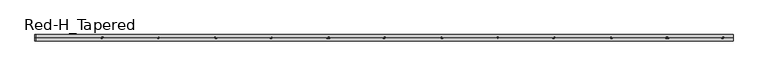
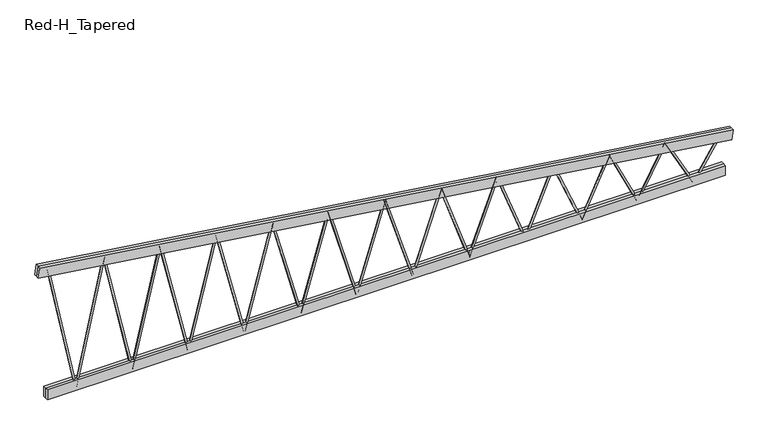
"""IFC4 building model written with IfcOpenShell, lengths in millimetres: beam geometry, Construction_Frames_RedBuilt_Openweb_Red-H_Tapered : Red-H_Tapered."""

from ifc_helpers import new_model, si_unit, point, frame, origin, origin_2d, place, context, project, spatial, polyline, circle_curve, trimmed, segment, composite_curve, outline, extrude, source, transform, mapped, element, save


def red_h_tapered_d8ccadf6(model_context):
    return source(origin(), model_context, "Body", "SweptSolid", [
        extrude(outline(composite_curve([segment(trimmed(circle_curve(origin_2d(), 12.7), [point((0.0, -12.7000001))], [point((0.0, 12.7))], False, "CARTESIAN"), True, "CONTINUOUS"), segment(trimmed(circle_curve(origin_2d(), 12.7), [point((0.0, 12.7))], [point((0.0, -12.7000001))], False, "CARTESIAN"), True, "CONTINUOUS")], self_intersect=False)), frame((-373.9223958, 0.0, -367.0101562), z_axis=(-0.2781430726229013, 0.0, 0.9605396562099305), x_axis=(0.0, -1.0, 0.0)), (0.0, 0.0, 1.0), 1344.3527186),
        extrude(outline(composite_curve([segment(trimmed(circle_curve(origin_2d(), 12.7), [point((0.0, 12.7))], [point((0.0, -12.7))], False, "CARTESIAN"), True, "CONTINUOUS"), segment(trimmed(circle_curve(origin_2d(), 12.7), [point((0.0, -12.7))], [point((0.0, 12.7))], False, "CARTESIAN"), True, "CONTINUOUS")], self_intersect=False)), frame((-1121.7671875, 0.0, -367.0101562), z_axis=(0.27814307262290183, 0.0, 0.9605396562099304), x_axis=(0.0, -1.0, 0.0)), (0.0, 0.0, 1.0), 1344.3527186),
        extrude(outline(composite_curve([segment(trimmed(circle_curve(origin_2d(), 12.7), [point((0.0, -12.7))], [point((0.0, 12.7))], False, "CARTESIAN"), True, "CONTINUOUS"), segment(trimmed(circle_curve(origin_2d(), 12.7), [point((0.0, 12.7))], [point((0.0, -12.7))], False, "CARTESIAN"), True, "CONTINUOUS")], self_intersect=False)), frame((-1121.7671875, 0.0, -367.0101562), z_axis=(-0.259370176676437, 0.0, 0.9657779824839837), x_axis=(0.0, -1.0, 0.0)), (0.0, 0.0, 1.0), 1441.655323),
        extrude(outline(composite_curve([segment(trimmed(circle_curve(origin_2d(), 12.7), [point((0.0, -12.6999999))], [point((0.0, 12.7))], False, "CARTESIAN"), True, "CONTINUOUS"), segment(trimmed(circle_curve(origin_2d(), 12.7), [point((0.0, 12.7))], [point((0.0, -12.6999999))], False, "CARTESIAN"), True, "CONTINUOUS")], self_intersect=False)), frame((-1869.6119792, 0.0, -367.0101562), z_axis=(0.2593701766764403, 0.0, 0.9657779824839828), x_axis=(0.0, -1.0, 0.0)), (0.0, 0.0, 1.0), 1441.655323),
        extrude(outline(composite_curve([segment(trimmed(circle_curve(origin_2d(), 12.7), [point((0.0, 12.7))], [point((0.0, -12.7))], False, "CARTESIAN"), True, "CONTINUOUS"), segment(trimmed(circle_curve(origin_2d(), 12.7), [point((0.0, -12.7))], [point((0.0, 12.7))], False, "CARTESIAN"), True, "CONTINUOUS")], self_intersect=False)), frame((-1869.6119792, 0.0, -367.0101562), z_axis=(-0.24289567030274667, 0.0, 0.970052417835335), x_axis=(0.0, -1.0, 0.0)), (0.0, 0.0, 1.0), 1539.4362335),
        extrude(outline(composite_curve([segment(trimmed(circle_curve(origin_2d(), 12.7), [point((0.0, -12.7))], [point((0.0, 12.7))], False, "CARTESIAN"), True, "CONTINUOUS"), segment(trimmed(circle_curve(origin_2d(), 12.7), [point((0.0, 12.7))], [point((0.0, -12.7))], False, "CARTESIAN"), True, "CONTINUOUS")], self_intersect=False)), frame((-2617.4567708, 0.0, -367.0101562), z_axis=(0.24289567030274511, 0.0, 0.9700524178353355), x_axis=(0.0, -1.0, 0.0)), (0.0, 0.0, 1.0), 1539.4362335),
        extrude(outline(composite_curve([segment(trimmed(circle_curve(origin_2d(), 12.7), [point((0.0, 12.6999999))], [point((0.0, -12.7))], False, "CARTESIAN"), True, "CONTINUOUS"), segment(trimmed(circle_curve(origin_2d(), 12.7), [point((0.0, -12.7))], [point((0.0, 12.6999999))], False, "CARTESIAN"), True, "CONTINUOUS")], self_intersect=False)), frame((-2617.4567708, 0.0, -367.0101562), z_axis=(-0.2283342477198344, 0.0, 0.9735828014700225), x_axis=(0.0, -1.0, 0.0)), (0.0, 0.0, 1.0), 1637.6097741),
        extrude(outline(composite_curve([segment(trimmed(circle_curve(origin_2d(), 12.7), [point((0.0, -12.7))], [point((0.0, 12.7))], False, "CARTESIAN"), True, "CONTINUOUS"), segment(trimmed(circle_curve(origin_2d(), 12.7), [point((0.0, 12.7))], [point((0.0, -12.7))], False, "CARTESIAN"), True, "CONTINUOUS")], self_intersect=False)), frame((-3365.3015625, 0.0, -367.0101562), z_axis=(0.22833424771983904, 0.0, 0.9735828014700214), x_axis=(0.0, -1.0, 0.0)), (0.0, 0.0, 1.0), 1637.6097741),
        extrude(outline(composite_curve([segment(trimmed(circle_curve(origin_2d(), 12.7), [point((0.0, 12.7))], [point((0.0, -12.7))], False, "CARTESIAN"), True, "CONTINUOUS"), segment(trimmed(circle_curve(origin_2d(), 12.7), [point((0.0, -12.7))], [point((0.0, 12.7))], False, "CARTESIAN"), True, "CONTINUOUS")], self_intersect=False)), frame((-3365.3015625, 0.0, -367.0101562), z_axis=(-0.215379519884342, 0.0, 0.9765304206292759), x_axis=(0.0, -1.0, 0.0)), (0.0, 0.0, 1.0), 1736.1093387),
        extrude(outline(composite_curve([segment(trimmed(circle_curve(origin_2d(), 12.7), [point((0.0, -12.7))], [point((0.0, 12.7000001))], False, "CARTESIAN"), True, "CONTINUOUS"), segment(trimmed(circle_curve(origin_2d(), 12.7), [point((0.0, 12.7000001))], [point((0.0, -12.7))], False, "CARTESIAN"), True, "CONTINUOUS")], self_intersect=False)), frame((-4113.1463542, 0.0, -367.0101562), z_axis=(0.21537951988434104, 0.0, 0.9765304206292761), x_axis=(0.0, -1.0, 0.0)), (0.0, 0.0, 1.0), 1736.1093387),
        extrude(outline(composite_curve([segment(trimmed(circle_curve(origin_2d(), 12.7), [point((0.0, 12.7))], [point((0.0, -12.7))], False, "CARTESIAN"), True, "CONTINUOUS"), segment(trimmed(circle_curve(origin_2d(), 12.7), [point((0.0, -12.7))], [point((0.0, 12.7))], False, "CARTESIAN"), True, "CONTINUOUS")], self_intersect=False)), frame((-4113.1463542, 0.0, -367.0101562), z_axis=(-0.20378548023403467, 0.0, 0.9790155657831922), x_axis=(0.0, -1.0, 0.0)), (0.0, 0.0, 1.0), 1834.8824234),
        extrude(outline(composite_curve([segment(trimmed(circle_curve(origin_2d(), 12.7), [point((0.0, 12.7))], [point((0.0, -12.7))], False, "CARTESIAN"), True, "CONTINUOUS"), segment(trimmed(circle_curve(origin_2d(), 12.7), [point((0.0, -12.7))], [point((0.0, 12.7))], False, "CARTESIAN"), True, "CONTINUOUS")], self_intersect=False)), frame((4113.1463542, 0.0, -367.0101562), z_axis=(0.5390888753862533, 0.0, 0.8422488850896657), x_axis=(0.0, -1.0, 0.0)), (0.0, 0.0, 1.0), 693.6192025),
        extrude(outline(composite_curve([segment(trimmed(circle_curve(origin_2d(), 12.7), [point((0.0, -12.7))], [point((0.0, 12.6999999))], False, "CARTESIAN"), True, "CONTINUOUS"), segment(trimmed(circle_curve(origin_2d(), 12.7), [point((0.0, 12.6999999))], [point((0.0, -12.7))], False, "CARTESIAN"), True, "CONTINUOUS")], self_intersect=False)), frame((4113.1463542, 0.0, -367.0101562), z_axis=(-0.47901881060106194, 0.0, 0.8778046360610908), x_axis=(0.0, -1.0, 0.0)), (0.0, 0.0, 1.0), 780.6006519),
        extrude(outline(composite_curve([segment(trimmed(circle_curve(origin_2d(), 12.7), [point((0.0, 12.7))], [point((0.0, -12.7))], False, "CARTESIAN"), True, "CONTINUOUS"), segment(trimmed(circle_curve(origin_2d(), 12.7), [point((0.0, -12.7))], [point((0.0, 12.7))], False, "CARTESIAN"), True, "CONTINUOUS")], self_intersect=False)), frame((3365.3015625, 0.0, -367.0101562), z_axis=(0.4790188106010647, 0.0, 0.8778046360610893), x_axis=(0.0, -1.0, 0.0)), (0.0, 0.0, 1.0), 780.6006519),
        extrude(outline(composite_curve([segment(trimmed(circle_curve(origin_2d(), 12.7), [point((0.0, -12.7))], [point((0.0, 12.7))], False, "CARTESIAN"), True, "CONTINUOUS"), segment(trimmed(circle_curve(origin_2d(), 12.7), [point((0.0, 12.7))], [point((0.0, -12.7))], False, "CARTESIAN"), True, "CONTINUOUS")], self_intersect=False)), frame((3365.3015625, 0.0, -367.0101562), z_axis=(-0.4294909226192341, 0.0, 0.9030711751504856), x_axis=(0.0, -1.0, 0.0)), (0.0, 0.0, 1.0), 870.6176921),
        extrude(outline(composite_curve([segment(trimmed(circle_curve(origin_2d(), 12.7), [point((0.0, 12.7000001))], [point((0.0, -12.7))], False, "CARTESIAN"), True, "CONTINUOUS"), segment(trimmed(circle_curve(origin_2d(), 12.7), [point((0.0, -12.7))], [point((0.0, 12.7000001))], False, "CARTESIAN"), True, "CONTINUOUS")], self_intersect=False)), frame((2617.4567708, 0.0, -367.0101562), z_axis=(0.42949092261923544, 0.0, 0.903071175150485), x_axis=(0.0, -1.0, 0.0)), (0.0, 0.0, 1.0), 870.6176921),
        extrude(outline(composite_curve([segment(trimmed(circle_curve(origin_2d(), 12.7), [point((0.0, -12.7))], [point((0.0, 12.7))], False, "CARTESIAN"), True, "CONTINUOUS"), segment(trimmed(circle_curve(origin_2d(), 12.7), [point((0.0, 12.7))], [point((0.0, -12.7))], False, "CARTESIAN"), True, "CONTINUOUS")], self_intersect=False)), frame((2617.4567708, 0.0, -367.0101562), z_axis=(-0.3883619744047195, 0.0, 0.9215069054741087), x_axis=(0.0, -1.0, 0.0)), (0.0, 0.0, 1.0), 962.8192781),
        extrude(outline(composite_curve([segment(trimmed(circle_curve(origin_2d(), 12.7), [point((0.0, 12.7))], [point((0.0, -12.7))], False, "CARTESIAN"), True, "CONTINUOUS"), segment(trimmed(circle_curve(origin_2d(), 12.7), [point((0.0, -12.7))], [point((0.0, 12.7))], False, "CARTESIAN"), True, "CONTINUOUS")], self_intersect=False)), frame((1869.6119792, 0.0, -367.0101562), z_axis=(0.38836197440472214, 0.0, 0.9215069054741076), x_axis=(0.0, -1.0, 0.0)), (0.0, 0.0, 1.0), 962.8192781),
        extrude(outline(composite_curve([segment(trimmed(circle_curve(origin_2d(), 12.7), [point((0.0, -12.7))], [point((0.0, 12.6999999))], False, "CARTESIAN"), True, "CONTINUOUS"), segment(trimmed(circle_curve(origin_2d(), 12.7), [point((0.0, 12.6999999))], [point((0.0, -12.7))], False, "CARTESIAN"), True, "CONTINUOUS")], self_intersect=False)), frame((1869.6119792, 0.0, -367.0101562), z_axis=(-0.3538808172794093, 0.0, 0.9352905255382722), x_axis=(0.0, -1.0, 0.0)), (0.0, 0.0, 1.0), 1056.6336958),
        extrude(outline(composite_curve([segment(trimmed(circle_curve(origin_2d(), 12.7), [point((0.0, 12.7))], [point((0.0, -12.7))], False, "CARTESIAN"), True, "CONTINUOUS"), segment(trimmed(circle_curve(origin_2d(), 12.7), [point((0.0, -12.7))], [point((0.0, 12.7))], False, "CARTESIAN"), True, "CONTINUOUS")], self_intersect=False)), frame((1121.7671875, 0.0, -367.0101562), z_axis=(0.3538808172794134, 0.0, 0.9352905255382706), x_axis=(0.0, -1.0, 0.0)), (0.0, 0.0, 1.0), 1056.6336958),
        extrude(outline(composite_curve([segment(trimmed(circle_curve(origin_2d(), 12.7), [point((0.0, -12.7))], [point((0.0, 12.7))], False, "CARTESIAN"), True, "CONTINUOUS"), segment(trimmed(circle_curve(origin_2d(), 12.7), [point((0.0, 12.7))], [point((0.0, -12.7))], False, "CARTESIAN"), True, "CONTINUOUS")], self_intersect=False)), frame((1121.7671875, 0.0, -367.0101562), z_axis=(-0.32467930219436536, 0.0, 0.9458241648036807), x_axis=(0.0, -1.0, 0.0)), (0.0, 0.0, 1.0), 1151.6668704),
        extrude(outline(composite_curve([segment(trimmed(circle_curve(origin_2d(), 12.7), [point((0.0, 12.7))], [point((0.0, -12.7))], False, "CARTESIAN"), True, "CONTINUOUS"), segment(trimmed(circle_curve(origin_2d(), 12.7), [point((0.0, -12.7))], [point((0.0, 12.7))], False, "CARTESIAN"), True, "CONTINUOUS")], self_intersect=False)), frame((373.9223958, 0.0, -367.0101562), z_axis=(0.3246793021943692, 0.0, 0.9458241648036794), x_axis=(0.0, -1.0, 0.0)), (0.0, 0.0, 1.0), 1151.6668704),
        extrude(outline(composite_curve([segment(trimmed(circle_curve(origin_2d(), 12.7), [point((0.0, -12.7))], [point((0.0, 12.7000001))], False, "CARTESIAN"), True, "CONTINUOUS"), segment(trimmed(circle_curve(origin_2d(), 12.7), [point((0.0, 12.7000001))], [point((0.0, -12.7))], False, "CARTESIAN"), True, "CONTINUOUS")], self_intersect=False)), frame((373.9223958, 0.0, -367.0101562), z_axis=(-0.299703677233337, 0.0, 0.9540323400455646), x_axis=(0.0, -1.0, 0.0)), (0.0, 0.0, 1.0), 1247.6403336),
        extrude(outline(composite_curve([segment(trimmed(circle_curve(origin_2d(), 12.7), [point((0.0, 12.7))], [point((0.0, -12.7000001))], False, "CARTESIAN"), True, "CONTINUOUS"), segment(trimmed(circle_curve(origin_2d(), 12.7), [point((0.0, -12.7000001))], [point((0.0, 12.7))], False, "CARTESIAN"), True, "CONTINUOUS")], self_intersect=False)), frame((-373.9223958, 0.0, -367.0101562), z_axis=(0.29970367723330027, 0.0, 0.9540323400455762), x_axis=(0.0, -1.0, 0.0)), (0.0, 0.0, 1.0), 1247.6403336),
        extrude(outline(polyline([(-4512.46875, -41.275), (-4512.46875, -3.175), (4512.46875, -3.175), (4512.46875, -41.275), (-4512.46875, -41.275)])), frame((0.0, 0.0, -386.0601562), z_axis=(0.0, 0.0, 1.0), x_axis=(1.0, 0.0, 0.0)), (0.0, 0.0, 1.0), 139.7),
        extrude(outline(polyline([(-4512.46875, 3.175), (-4512.46875, 41.275), (4512.46875, 41.275), (4512.46875, 3.175), (-4512.46875, 3.175)])), frame((0.0, 0.0, -386.0601562), z_axis=(0.0, 0.0, 1.0), x_axis=(1.0, 0.0, 0.0)), (0.0, 0.0, 1.0), 139.7),
        extrude(outline(polyline([(0.0, -38.1), (0.0, 0.0), (9316.8578936, 0.0), (9316.8578936, -38.1), (0.0, -38.1)])), frame((-4633.3019713, -3.175, 1367.8701462), z_axis=(0.13767517060507875, 0.0, 0.9904774340684711), x_axis=(0.9904774340684711, 0.0, -0.13767517060507875)), (0.0, 0.0, 1.0), 139.7),
        extrude(outline(polyline([(0.0, -38.1), (0.0, 0.0), (9316.8578936, 0.0), (9316.8578936, -38.1), (0.0, -38.1)])), frame((-4633.3019713, 41.275, 1367.8701462), z_axis=(0.13767517060507875, 0.0, 0.9904774340684711), x_axis=(0.9904774340684711, 0.0, -0.13767517060507875)), (0.0, 0.0, 1.0), 139.7),
    ])


if __name__ == "__main__":
    model = new_model("IFC4")
    model_context = context("Model", 3, world=origin())
    ifc_project = project(units=[si_unit("LENGTHUNIT", "METRE", prefix="MILLI")], contexts=[model_context])
    site = spatial("IfcSite", under=ifc_project)
    building = spatial("IfcBuilding", under=site)
    placement = place(None, origin())
    red_h_tapered_shape = red_h_tapered_d8ccadf6(model_context)
    element("IfcBeam", 1, ObjectType="Construction_Frames_RedBuilt_Openweb_Red-H_Tapered : Red-H_Tapered", at=placement, inside=building, context=model_context, shape_type="MappedRepresentation", body=[
        mapped(red_h_tapered_shape, transform((0.0, 0.0, 0.0), x_axis=(1.0, 0.0, 0.0), y_axis=(0.0, 1.0, 0.0), z_axis=(0.0, 0.0, 1.0))),
    ])
    save(model, "model.ifc")

# Revit data of these elements
# Type "Construction_Frames_RedBuilt_Openweb_Red-H_Tapered : Red-H_Tapered"
#   Youtube clip = ""
#   Weight Net (Kg) = "0"
#   Webs = "Up to 2\" diameter tubular steel"
#   Uniformat II Description = ""
#   Uniformat II Code = ""
#   Uniclass 2015 Name = "Softwood trusses"
#   Uniclass 2015 Code = "Pr_20_85_90_81"
#   Uniclass 2.0 Description = "Structural Framing Systems"
#   Uniclass 2.0 Code = "SS-15-10-75"
#   Uniclass 1.4 Description = "Trusses"
#   Uniclass 1.4 Code = "L3523"
#   UNSPSC Code = "30103606"
#   Technical description = "http://www.redbuilt.com/reference/literature-and-other-resources"
#   Region South America = "None"
#   Region Oceania = "None"
#   Region North America = "US"
#   Region Middle East = "None"
#   Region Europe = "None"
#   Region Asia = "None"
#   Region Antarctica = "None"
#   Region Africa = "None"
#   QR code = "http://bimobject.com/redbuilt/product/redbuilt-0003"
#   Product url = "http://www.redbuilt.com/products/default.aspx?id=2"
#   Product group = "Wood Trusses"
#   Product family = "Construction"
#   Product data url = "https://bimobject.com/redbuilt/product/redbuilt-0003"
#   Product certification = ""
#   Product SKU = "redbuilt-0003"
#   Product Page URL = "http://www.redbuilt.com/commercial-systems/red-m-red-h-open-web-trusses"
#   Product Guid = "2c5793f2-6ffb-4665-b825-cf90c048e711"
#   Product Documentation Link = "http://www.redbuilt.com/documents/OW_Guide_2017_07_LowRes_wLinks.pdf"
#   OmniClass Description = "Wood Trusses"
#   OmniClass Code = "23-13 35 19 13 17"
#   NBS Reference Description = ""
#   NBS Reference Code = ""
#   Material secondary = "Steel"
#   Material main = "Wood"
#   Masterformat 2014 Description = "Metal-Web Wood Joists"
#   Masterformat 2014 Code = "06 17 36"
#   Manufacturer name = "RedBuilt"
#   Manufacturer country = "United States"
#   Installation instructions = "http://www.redbuilt.com/documents/Installation_Sheets_Open-Web.pdf"
#   IFC Classification = ""
#   EAN code = ""
#   Design country = "United States"
#   Product Information = "http://redbuilt.com/products/default.aspx?id=2"
#   Model = "Red-H-Tapered"
#   Manufacturer URL = "http://redbuilt.com/"
#   Manufacturer = "RedBuilt™"
#   Description = "Open Web Truss"
#   Date of publishing = "8/17/2010"
#   Contact us = "http://redbuilt.com/contact/"
#   Chords = "Double 1½\" x 5½\" MSR lumber"
#   COBIe Type Category = ""
#   Brand url = "http://www.redbuilt.com"
#   BIMobject main category code = "construction"
#   BIMobject main category = "Construction"
#   BIMobject category code = "construction-frames-trusses"
#   BIMobject category = "Frames & Trusses"
#   Web Radius = 0' - 0 1/2"
#   Web Layout Offset Start [instance default] = 0' - 5"
#   Web Layout Offset End [instance default] = 0' - 5"
#   Web Diameter = 0' - 1"
#   TotalLength [instance default] = 20' - 0"
#   Span Minimum = 4' - 0"
#   Span Maximum = 70' - 0"
#   Span Limit [instance default] = 20' - 0"
#   Nominal width = 0' - 0"
#   Nominal height = 0' - 0"
#   Inner Depth Top [instance default] = 0' - 2.76372"
#   Depth Start [instance default] = 6' - 0"
#   Top Chord Length [instance default] = 20' - 1.19701"
#   TC Extension Start Aux [instance default] = 0' - 0"
#   TC Extension End Aux [instance default] = 0' - 0"
#   T-B Chord Length Difference L [instance default] = 0' - 4"
#   T-B Chord Length Difference [instance default] = 0' - 4"
#   Height 2 [instance default] = 6' - 0"
#   Depth Minimum at Wall = 2' - 0"
#   Depth Maximum at Wall = 6' - 0"
#   Depth Lower End [instance default] = 2' - 0"
#   Depth Higher End [instance default] = 6' - 0"
#   Depth End [instance default] = 2' - 0"
#   Depth 2 [instance default] = 2' - 0"
#   Chord Width = 0' - 3 1/4"
#   Chord Thickness = 0' - 1 1/2"
#   Chord Depth = 0' - 5 1/2"
#   Offset Start [instance default] = 0' - 0"
#   TC Extension Start [instance default] = 0' - 0"
#   End Panel = 0' - 5"
#   Offset End [instance default] = 0' - 0"
#   TC Extension End [instance default] = 0' - 0"
#   Length [instance default] = 20' - 0"
#   Angle [instance default] = 5.71059°
#   Span Limit Warning [instance default] = no
#   Edition number = 1
#   Top Bearing Start [instance default] = yes
#   Top Bearing End [instance default] = yes
#   Bottom Bearing Start [instance default] = no
#   Bottom Bearing End [instance default] = no
#   8 Panels [instance default] = yes
#   16 Panels [instance default] = no
#   12 Panels [instance default] = no
#   Web Material = RedBuilt-Steel, Galvanized
#   Clip Material = RedBuilt-Steel, Galvanized
#   Chords Material = RedBuilt-MSR
#   URL = ""
#   Assembly Code = ""
# Element 1 (IfcBeam, "Construction_Frames_RedBuilt_Openweb_Red-H_Tapered : Red-H_Tapered")
#   TotalLength = 30' - 3 5/16"
#   Span Limit = 30' - 3 5/16"
#   Inner Depth Top = 0' - 2.77644"
#   Top Chord Length = 30' - 6.80543"
#   Depth 2 = 4' - 2 1/2"
#   Angle = 7.91334°
#   8 Panels = no
#   12 Panels = yes
#   Materials on its faces: "RedBuilt-Steel, Galvanized", "RedBuilt-MSR"
# Materials
#   "RedBuilt-Steel, Galvanized": class "Metal", colour RGB 164 172 176, transparency 0, Manufacturer = "RedBuilt. LLC", Comments = "Openweb Metal Web", URL = "http://www.redbuilt.com/", Description = "Galvanized steel", Cost = 0
#   "RedBuilt-MSR": class "Wood", colour RGB 213 182 136, transparency 0, Manufacturer = "RedBuilt, LLC", URL = "http://www.redbuilt.com/", Cost = 0
